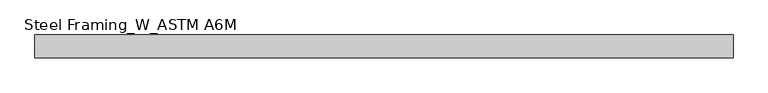
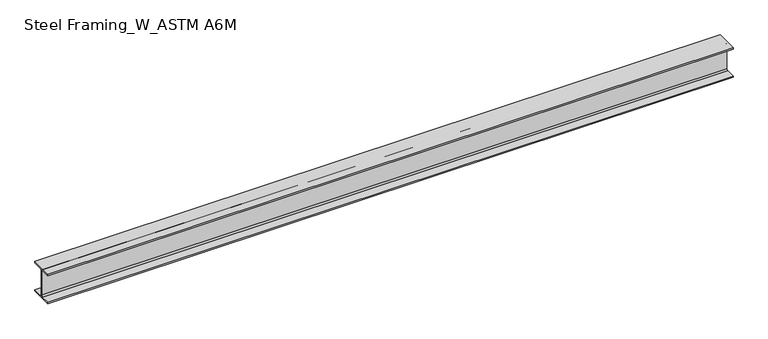
"""IFC4 building model written with IfcOpenShell, lengths in millimetres: beam geometry, Steel Framing_W_ASTM A6M : H_SB_AR_S02_W360x91_B3."""

from ifc_helpers import new_model, si_unit, point, frame, frame_2d, origin, place, context, project, spatial, polyline, circle_curve, trimmed, segment, composite_curve, outline, extrude, source, transform, mapped, element, save


def steel_framing_w_astm_a6m_977104bc(model_context):
    return source(origin(), model_context, "Body", "SweptSolid", [
        extrude(outline(composite_curve([segment(polyline([(127.0, -160.1), (127.0, -176.5), (-127.0, -176.5), (-127.0, -160.1), (-19.865, -160.1)]), True, "CONTINUOUS"), segment(trimmed(circle_curve(frame_2d((-19.865, -145.0)), 15.1), [point((-19.865, -160.1))], [point((-4.765, -145.0))], True, "CARTESIAN"), True, "CONTINUOUS"), segment(polyline([(-4.765, -145.0), (-4.765, 145.0)]), True, "CONTINUOUS"), segment(trimmed(circle_curve(frame_2d((-19.865, 145.0)), 15.1), [point((-4.765, 145.0))], [point((-19.865, 160.1))], True, "CARTESIAN"), True, "CONTINUOUS"), segment(polyline([(-19.865, 160.1), (-127.0, 160.1), (-127.0, 176.5), (127.0, 176.5), (127.0, 160.1), (19.865, 160.1)]), True, "CONTINUOUS"), segment(trimmed(circle_curve(frame_2d((19.865, 145.0)), 15.1), [point((19.865, 160.1))], [point((4.765, 145.0))], True, "CARTESIAN"), True, "CONTINUOUS"), segment(polyline([(4.765, 145.0), (4.765, -145.0)]), True, "CONTINUOUS"), segment(trimmed(circle_curve(frame_2d((19.865, -145.0)), 15.1), [point((4.765, -145.0))], [point((19.865, -160.1))], True, "CARTESIAN"), True, "CONTINUOUS"), segment(polyline([(19.865, -160.1), (127.0, -160.1)]), True, "CONTINUOUS")], self_intersect=False)), frame((-3860.3, 0.0, 0.0), z_axis=(1.0, 0.0, 0.0), x_axis=(0.0, 1.0, 0.0)), (0.0, 0.0, 1.0), 7720.6),
    ])


if __name__ == "__main__":
    model = new_model("IFC4")
    model_context = context("Model", 3, world=origin())
    ifc_project = project(units=[si_unit("LENGTHUNIT", "METRE", prefix="MILLI")], contexts=[model_context])
    site = spatial("IfcSite", under=ifc_project)
    building = spatial("IfcBuilding", under=site)
    placement = place(None, origin())
    steel_framing_w_astm_a6m_shape = steel_framing_w_astm_a6m_977104bc(model_context)
    element("IfcBeam", 1, ObjectType="Steel Framing_W_ASTM A6M : H_SB_AR_S02_W360x91_B3", at=placement, inside=building, context=model_context, shape_type="MappedRepresentation", body=[
        mapped(steel_framing_w_astm_a6m_shape, transform((0.0, 0.0, 0.0), x_axis=(1.0, 0.0, 0.0), y_axis=(0.0, 1.0, 0.0), z_axis=(0.0, 0.0, 1.0))),
    ])
    save(model, "model.ifc")

# Revit data of these elements
# Type "Steel Framing_W_ASTM A6M : H_SB_AR_S02_W360x91_B3"
#   Type Mark = "B3"
#   Section Name Key = "W14x61"
#   Width = 25.4 cm
#   Web Thickness = 0.953 cm
#   Web Fillet = 1.51 cm
#   Warping Constant = 1260000.0 cm⁶
#   Torsional Moment of Inertia = 91.20 cm⁴
#   Section Area = 115.0 cm²
#   Plastic Modulus weak axis = 537.0 cm³
#   Plastic Modulus strong axis = 1670.0 cm³
#   Perimeter = 1.68 m²/m
#   Nominal Weight = 91.00 kgf/m
#   Moment of Inertia weak axis = 4450.00 cm⁴
#   Moment of Inertia strong axis = 26600.00 cm⁴
#   Height = 35.3 cm
#   Flange Thickness = 1.64 cm
#   Elastic Modulus weak axis = 352.0 cm³
#   Elastic Modulus strong axis = 1510.0 cm³
#   Centroid Vertical = 17.65 cm
#   Centroid Horizontal = 12.7 cm
#   Length [instance default] = 1500 mm
#   Structural Material [instance default] = Steel, 45-345
#   Bolt Spacing = 0
#   Assembly Code = ""
# Element 1 (IfcBeam, "Steel Framing_W_ASTM A6M : H_SB_AR_S02_W360x91_B3")
#   Materials on its faces: "Steel, 45-345"
# Materials
#   "Steel, 45-345": class "Metal", colour RGB 189 187 185, transparency 0, Description = "Steel 345 MPa", Cost = 0
